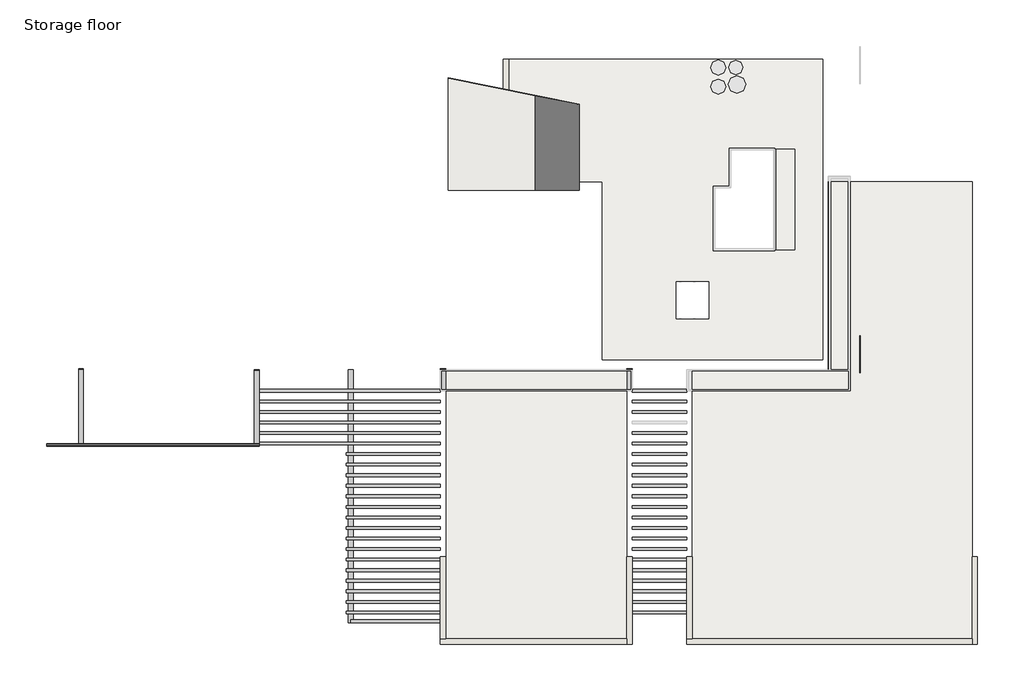
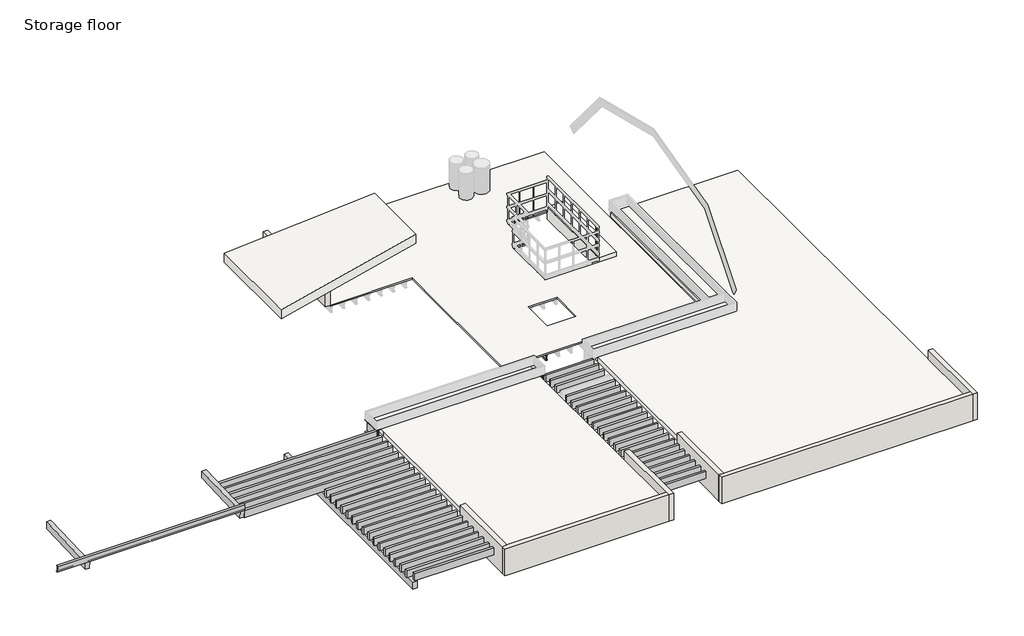
# One storey, part 1 of 2: 54 beams, 7 walls, 4 slabs, 1 roof.
"""IFC4 building model written with IfcOpenShell, lengths in millimetres."""

import ifcopenshell
import ifcopenshell.guid

model = None  # the IFC model being written
_history = None  # IfcOwnerHistory: only IFC2X3 demands one
_inside = {}  # id of a spatial element -> (the spatial element, [elements in it])
_under = {}  # id of a project, library or spatial element -> (it, [spatial elements below it])
_declared = {}  # id of a project -> (the project, [libraries it declares])
_typed = {}  # id of a type object -> (the type object, [elements of that type])
_made_of = {}  # id of a material, layer set ... -> (it, [elements and type objects made of it])


def new_model(schema):
    """Start an empty IFC model of exactly this schema.

    Asked for "IFC4X3", IfcOpenShell would pick the latest addendum, in which some entities
    have other attributes; the version numbers below select the first issue.
    IFC2X3 requires an IfcOwnerHistory on every rooted entity: one is made here for all.
    """
    global model, _history
    if schema == "IFC4X3":
        model = ifcopenshell.file(schema_version=(4, 3, 0, 0))
    else:
        model = ifcopenshell.file(schema=schema)
    _inside.clear()
    _under.clear()
    _declared.clear()
    _typed.clear()
    _made_of.clear()
    _history = None
    if model.schema == "IFC2X3":
        org = make("IfcOrganization", Name="unknown")
        user = make(
            "IfcPersonAndOrganization",
            ThePerson=make("IfcPerson", FamilyName="unknown"),
            TheOrganization=org,
        )
        app = make(
            "IfcApplication",
            ApplicationDeveloper=org,
            Version="unknown",
            ApplicationFullName="unknown",
            ApplicationIdentifier="unknown",
        )
        _history = make(
            "IfcOwnerHistory",
            OwningUser=user,
            OwningApplication=app,
            ChangeAction="ADDED",
            CreationDate=0,
        )
    return model


def make(cls, **values):
    """One entity of the class cls with the attributes given. An attribute that is None is left unset."""
    return model.create_entity(
        cls, **{name: value for name, value in values.items() if value is not None}
    )


def rooted(cls, **values):
    """An entity with a GlobalId (a new one), such as an element, a storey or a relation."""
    return make(cls, GlobalId=ifcopenshell.guid.new(), OwnerHistory=_history, **values)


def si_unit(unit_type, name, prefix=None):
    """IfcSIUnit, for example si_unit("LENGTHUNIT", "METRE", prefix="MILLI")."""
    return make("IfcSIUnit", UnitType=unit_type, Prefix=prefix, Name=name)


def assignment(units):
    """IfcUnitAssignment: the units of a project."""
    return None if units is None else make("IfcUnitAssignment", Units=units)


def point(xyz):
    """IfcCartesianPoint."""
    return None if xyz is None else make("IfcCartesianPoint", Coordinates=xyz)


def direction(xyz):
    """IfcDirection."""
    return None if xyz is None else make("IfcDirection", DirectionRatios=xyz)


def frame(location, z_axis=None, x_axis=None):
    """IfcAxis2Placement3D, a coordinate frame: its origin and axes. An axis left out is left unset."""
    return make(
        "IfcAxis2Placement3D",
        Location=point(location),
        Axis=direction(z_axis),
        RefDirection=direction(x_axis),
    )


def frame_2d(location, x_axis=None):
    """IfcAxis2Placement2D, a coordinate frame in the plane: its origin and x axis."""
    return make(
        "IfcAxis2Placement2D", Location=point(location), RefDirection=direction(x_axis)
    )


def origin():
    """The frame at (0, 0, 0) with its axes left unset."""
    return frame((0.0, 0.0, 0.0))


def place(relative_to, where):
    """IfcLocalPlacement: puts the frame where relative to a parent placement (None: the world)."""
    return make(
        "IfcLocalPlacement", PlacementRelTo=relative_to, RelativePlacement=where
    )


def context(
    kind, dimensions, precision=None, world=None, true_north=None, identifier=None
):
    """IfcGeometricRepresentationContext, for example the 3D "Model" context."""
    return make(
        "IfcGeometricRepresentationContext",
        ContextIdentifier=identifier,
        ContextType=kind,
        CoordinateSpaceDimension=dimensions,
        Precision=precision,
        WorldCoordinateSystem=world,
        TrueNorth=true_north,
    )


def project(units=None, contexts=None):
    """IfcProject with its units and contexts."""
    return rooted(
        "IfcProject",
        Name="project",
        RepresentationContexts=contexts,
        UnitsInContext=assignment(units),
    )


def spatial(cls, under=None, at=None, **own):
    """A site, building, storey or space (cls), placed at a placement, below another one or the project."""
    s = rooted(cls, ObjectPlacement=at, **own)
    if under is not None:
        _under.setdefault(under.id(), (under, []))[1].append(s)
    return s


def polyline(points):
    """IfcPolyline through the points."""
    return make("IfcPolyline", Points=[point(p) for p in points])


def circle_curve(where, radius):
    """IfcCircle in the frame where."""
    return make("IfcCircle", Position=where, Radius=radius)


def trimmed(basis, trim1, trim2, sense, master):
    """IfcTrimmedCurve: the piece of a basis curve between two trims."""
    return make(
        "IfcTrimmedCurve",
        BasisCurve=basis,
        Trim1=trim1,
        Trim2=trim2,
        SenseAgreement=sense,
        MasterRepresentation=master,
    )


def segment(curve, same_sense, transition):
    """IfcCompositeCurveSegment."""
    return make(
        "IfcCompositeCurveSegment",
        Transition=transition,
        SameSense=same_sense,
        ParentCurve=curve,
    )


def composite_curve(segments, self_intersect=None):
    """IfcCompositeCurve: segments joined end to end."""
    return make("IfcCompositeCurve", Segments=segments, SelfIntersect=self_intersect)


def outline(outer, holes=None, kind="AREA"):
    """IfcArbitraryClosedProfileDef: a profile drawn as a closed curve; with holes, ...WithVoids."""
    if holes is None:
        return make("IfcArbitraryClosedProfileDef", ProfileType=kind, OuterCurve=outer)
    return make(
        "IfcArbitraryProfileDefWithVoids",
        ProfileType=kind,
        OuterCurve=outer,
        InnerCurves=holes,
    )


def extrude(swept, where, along, depth):
    """IfcExtrudedAreaSolid: the profile swept, set in the frame where, extruded along a direction by depth."""
    return make(
        "IfcExtrudedAreaSolid",
        SweptArea=swept,
        Position=where,
        ExtrudedDirection=direction(along),
        Depth=depth,
    )


def faces_of(points, faces, orient=None, outer=None):
    """IfcFace entities. A face is a list of loops; a loop is a list of indices into points, from 0.

    orient and outer hold one flag for each loop. By default every Orientation is true, the
    first loop of a face is its IfcFaceOuterBound and the others are IfcFaceBound.
    """
    made = []
    for i, loops in enumerate(faces):
        bounds = []
        for j, loop in enumerate(loops):
            is_outer = j == 0 if outer is None else outer[i][j]
            bounds.append(
                make(
                    "IfcFaceOuterBound" if is_outer else "IfcFaceBound",
                    Bound=make("IfcPolyLoop", Polygon=[points[k] for k in loop]),
                    Orientation=True if orient is None else orient[i][j],
                )
            )
        made.append(make("IfcFace", Bounds=bounds))
    return made


def faceted_brep(points, faces, orient=None, outer=None, voids=None):
    """IfcFacetedBrep: a solid bounded by flat faces; with voids (closed shells), ...WithVoids."""
    shared = [point(p) for p in points]
    hull = make("IfcClosedShell", CfsFaces=faces_of(shared, faces, orient, outer))
    if voids is None:
        return make("IfcFacetedBrep", Outer=hull)
    return make(
        "IfcFacetedBrepWithVoids",
        Outer=hull,
        Voids=[
            make(cls, CfsFaces=faces_of(shared, fs, o, b)) for cls, fs, o, b in voids
        ],
    )


def shape(context_of_items, identifier, shape_type, items):
    """IfcShapeRepresentation: the items that make up one representation, for example the "Body"."""
    return make(
        "IfcShapeRepresentation",
        ContextOfItems=context_of_items,
        RepresentationIdentifier=identifier,
        RepresentationType=shape_type,
        Items=items,
    )


def source(mapping_origin, context_of_items, identifier, shape_type, items):
    """IfcRepresentationMap: a shape defined once, which mapped items show again and again."""
    return make(
        "IfcRepresentationMap",
        MappingOrigin=mapping_origin,
        MappedRepresentation=shape(context_of_items, identifier, shape_type, items),
    )


def transform(
    local_origin,
    x_axis=None,
    y_axis=None,
    z_axis=None,
    scale=None,
    scale2=None,
    scale3=None,
    uniform=True,
):
    """IfcCartesianTransformationOperator3D, or its non-uniform kind. x_axis, y_axis, z_axis: its Axis1, 2, 3."""
    if uniform:
        return make(
            "IfcCartesianTransformationOperator3D",
            Axis1=direction(x_axis),
            Axis2=direction(y_axis),
            LocalOrigin=point(local_origin),
            Scale=scale,
            Axis3=direction(z_axis),
        )
    return make(
        "IfcCartesianTransformationOperator3DnonUniform",
        Axis1=direction(x_axis),
        Axis2=direction(y_axis),
        LocalOrigin=point(local_origin),
        Scale=scale,
        Axis3=direction(z_axis),
        Scale2=scale2,
        Scale3=scale3,
    )


def mapped(mapping_source, mapping_target):
    """IfcMappedItem: shows the shape of a source again, moved by a transform."""
    return make(
        "IfcMappedItem", MappingSource=mapping_source, MappingTarget=mapping_target
    )


def made_of(thing, what):
    """Note that an element or type object is made of a material, layer set ...; save() writes the relation."""
    if what is not None:
        _made_of.setdefault(what.id(), (what, []))[1].append(thing)
    return thing


def element(
    cls,
    number,
    at=None,
    inside=None,
    cuts=None,
    type_object=None,
    material=None,
    context=None,
    identifier="Body",
    shape_type=None,
    held_by="IfcProductDefinitionShape",
    body=None,
    shapes=None,
    **own,
):
    """One element of the class cls, such as IfcWall. Its Tag is "e" and its number.

    at: its placement. inside: the storey or other place that contains it. cuts: it is an
    opening in that element (IfcRelVoidsElement). A single representation is given by context,
    identifier, shape_type and body (its items); several are given by shapes. held_by: the class
    of the entity that holds the representations. save() writes the other relations.
    """
    e = rooted(cls, Tag="e%d" % number, ObjectPlacement=at, **own)
    if body is not None:
        shapes = [shape(context, identifier, shape_type, body)]
    if shapes is not None:
        e.Representation = make(held_by, Representations=shapes)
    if inside is not None:
        _inside.setdefault(inside.id(), (inside, []))[1].append(e)
    if cuts is not None:
        rooted(
            "IfcRelVoidsElement", RelatingBuildingElement=cuts, RelatedOpeningElement=e
        )
    if type_object is not None:
        _typed.setdefault(type_object.id(), (type_object, []))[1].append(e)
    return made_of(e, material)


def aggregate(whole, parts):
    """IfcRelAggregates: a whole, such as a stair, and the parts it consists of."""
    return rooted("IfcRelAggregates", RelatingObject=whole, RelatedObjects=parts)


def save(model, path):
    """Write the relations noted so far, then the file.

    IfcRelAggregates (storeys below a building ...), IfcRelContainedInSpatialStructure (elements
    in a storey), IfcRelDefinesByType, IfcRelAssociatesMaterial and IfcRelDeclares: one each for
    every whole, place, type object, material and project.
    """
    for whole, parts in _under.values():
        aggregate(whole, parts)
    for where, things in _inside.values():
        rooted(
            "IfcRelContainedInSpatialStructure",
            RelatedElements=things,
            RelatingStructure=where,
        )
    for kind, things in _typed.values():
        rooted("IfcRelDefinesByType", RelatedObjects=things, RelatingType=kind)
    for what, things in _made_of.values():
        rooted("IfcRelAssociatesMaterial", RelatedObjects=things, RelatingMaterial=what)
    for by, libraries in _declared.values():
        rooted("IfcRelDeclares", RelatingContext=by, RelatedDefinitions=libraries)
    model.write(path)


def c_channel_c_3x8_0f191833(model_context):
    return source(origin(), model_context, "Body", "SweptSolid", [
        extrude(outline(composite_curve([segment(polyline([(-13.5128, 101.6), (44.9072, 101.6)]), True, "CONTINUOUS"), segment(trimmed(circle_curve(frame_2d((35.6108, 101.6)), 9.2964), [point((44.9072, 101.6))], [point((35.6108, 92.3036))], False, "CARTESIAN"), True, "CONTINUOUS"), segment(polyline([(35.6108, 92.3036), (-2.8702, 86.2088084), (-2.8702, -86.2088084), (35.6108, -92.3036)]), True, "CONTINUOUS"), segment(trimmed(circle_curve(frame_2d((35.6108, -101.6)), 9.2964), [point((35.6108, -92.3036))], [point((44.9072, -101.6))], False, "CARTESIAN"), True, "CONTINUOUS"), segment(polyline([(44.9072, -101.6), (-13.5128, -101.6), (-13.5128, 101.6)]), True, "CONTINUOUS")], self_intersect=False)), frame((-12252.325, 0.0, 0.0), z_axis=(1.0, 0.0, 0.0), x_axis=(0.0, 1.0, 0.0)), (0.0, 0.0, 1.0), 6108.7),
    ])


def plywood_web_joist_2_x_8_7c958bd9(model_context):
    return source(origin(), model_context, "Body", "SweptSolid", [
        extrude(outline(polyline([(-25.4, 101.6), (25.4, 101.6), (25.4, 63.5), (4.7625, 63.5), (4.7625, 69.85), (-4.7625, 69.85), (-4.7625, 63.5), (-25.4, 63.5), (-25.4, 101.6)])), frame((-4318.0, 0.0, 0.0), z_axis=(1.0, 0.0, 0.0), x_axis=(0.0, 1.0, 0.0)), (0.0, 0.0, 1.0), 8636.0),
        extrude(outline(polyline([(25.4, -63.5), (25.4, -101.6), (-25.4, -101.6), (-25.4, -63.5), (-4.7625, -63.5), (-4.7625, -69.1160374), (4.7625, -69.1160374), (4.7625, -63.5), (25.4, -63.5)])), frame((-4318.0, 0.0, 0.0), z_axis=(1.0, 0.0, 0.0), x_axis=(0.0, 1.0, 0.0)), (0.0, 0.0, 1.0), 8636.0),
        extrude(outline(polyline([(4318.0, 4.7625), (4318.0, -4.7625), (-4318.0, -4.7625), (-4318.0, 4.7625), (4318.0, 4.7625)])), frame((0.0, 0.0, -69.1160374), z_axis=(0.0, 0.0, 1.0), x_axis=(1.0, 0.0, 0.0)), (0.0, 0.0, 1.0), 138.9660374),
    ])


def timber_3x10_5e682144(model_context):
    return source(origin(), model_context, "Body", "SweptSolid", [
        extrude(outline(polyline([(1352.55, 38.1), (1352.55, -38.1), (-1352.55, -38.1), (-1352.55, 38.1), (1352.55, 38.1)])), frame((0.0, 0.0, -120.65), z_axis=(0.0, 0.0, 1.0), x_axis=(1.0, 0.0, 0.0)), (0.0, 0.0, 1.0), 241.3),
    ])


def timber_3x10_88a0bdfd(model_context):
    return source(origin(), model_context, "Body", "SweptSolid", [
        extrude(outline(polyline([(785.1325751, 38.1), (785.1325751, -38.1), (-785.1325751, -38.1), (-785.1325751, 38.1), (785.1325751, 38.1)])), frame((0.0, 0.0, -120.65), z_axis=(0.0, 0.0, 1.0), x_axis=(1.0, 0.0, 0.0)), (0.0, 0.0, 1.0), 241.3),
    ])


def timber_3x10_fcfe8c29(model_context):
    return source(origin(), model_context, "Body", "SweptSolid", [
        extrude(outline(polyline([(2603.5, 38.1), (2603.5, -38.1), (-2603.5, -38.1), (-2603.5, 38.1), (2603.5, 38.1)])), frame((0.0, 0.0, -120.65), z_axis=(0.0, 0.0, 1.0), x_axis=(1.0, 0.0, 0.0)), (0.0, 0.0, 1.0), 241.3),
    ])


def timber_3x10_eec112f8(model_context):
    return source(origin(), model_context, "Body", "SweptSolid", [
        extrude(outline(polyline([(2565.4, 38.1), (2565.4, -38.1), (-2641.6, -38.1), (-2641.6, 38.1), (2565.4, 38.1)])), frame((0.0, 0.0, -120.65), z_axis=(0.0, 0.0, 1.0), x_axis=(1.0, 0.0, 0.0)), (0.0, 0.0, 1.0), 241.3),
    ])


def timber_3x10_b3201cc8(model_context):
    return source(origin(), model_context, "Body", "SweptSolid", [
        extrude(outline(polyline([(1384.2999994, 38.1), (1384.2999994, -38.1), (-1197.0684633, -38.1), (-1197.0684633, 38.1), (1384.2999994, 38.1)])), frame((0.0, 0.0, -120.65), z_axis=(0.0, 0.0, 1.0), x_axis=(1.0, 0.0, 0.0)), (0.0, 0.0, 1.0), 241.3),
    ])


def timber_6x10_702de74f(model_context):
    return source(origin(), model_context, "Body", "SweptSolid", [
        extrude(outline(polyline([(1096.3279, 69.85), (1096.3279, -69.85), (-1065.1814977, -69.85), (-1065.1814977, 69.85), (1096.3279, 69.85)])), frame((0.0, 0.0, -120.65), z_axis=(0.0, 0.0, 1.0), x_axis=(1.0, 0.0, 0.0)), (0.0, 0.0, 1.0), 241.3),
    ])


def timber_6x10_97aa413e(model_context):
    return source(origin(), model_context, "Body", "SweptSolid", [
        extrude(outline(polyline([(1096.3279, 69.85), (1096.3279, -69.85), (-1091.5816749, -69.85), (-1091.5816749, 69.85), (1096.3279, 69.85)])), frame((0.0, 0.0, -120.65), z_axis=(0.0, 0.0, 1.0), x_axis=(1.0, 0.0, 0.0)), (0.0, 0.0, 1.0), 241.3),
    ])


def timber_6x10_01175893(model_context):
    return source(origin(), model_context, "Body", "SweptSolid", [
        extrude(outline(polyline([(1821.0853, 69.85), (1821.0853, -69.85), (-5454.65, -69.85), (-5454.65, 69.85), (1821.0853, 69.85)])), frame((0.0, 0.0, -120.65), z_axis=(0.0, 0.0, 1.0), x_axis=(1.0, 0.0, 0.0)), (0.0, 0.0, 1.0), 241.3),
    ])


def w_shapes_w_6x16_3_4_094122b6(model_context):
    return source(origin(), model_context, "Body", "SweptSolid", [
        extrude(outline(composite_curve([segment(polyline([(76.1964281, -203.073), (76.1964281, -212.725), (-76.2035719, -212.725), (-76.2035719, -203.073), (-10.5445719, -203.073)]), True, "CONTINUOUS"), segment(trimmed(circle_curve(frame_2d((-10.5445719, -195.453)), 7.62), [point((-10.5445719, -203.073))], [point((-2.9245719, -195.453))], True, "CARTESIAN"), True, "CONTINUOUS"), segment(polyline([(-2.9245719, -195.453), (-2.9245719, 195.453)]), True, "CONTINUOUS"), segment(trimmed(circle_curve(frame_2d((-10.5445719, 195.453)), 7.62), [point((-2.9245719, 195.453))], [point((-10.5445719, 203.073))], True, "CARTESIAN"), True, "CONTINUOUS"), segment(polyline([(-10.5445719, 203.073), (-76.2035719, 203.073), (-76.2035719, 212.725), (76.1964281, 212.725), (76.1964281, 203.073), (10.5374281, 203.073)]), True, "CONTINUOUS"), segment(trimmed(circle_curve(frame_2d((10.5374281, 195.453)), 7.62), [point((10.5374281, 203.073))], [point((2.9174281, 195.453))], True, "CARTESIAN"), True, "CONTINUOUS"), segment(polyline([(2.9174281, 195.453), (2.9174281, -195.453)]), True, "CONTINUOUS"), segment(trimmed(circle_curve(frame_2d((10.5374281, -195.453)), 7.62), [point((2.9174281, -195.453))], [point((10.5374281, -203.073))], True, "CARTESIAN"), True, "CONTINUOUS"), segment(polyline([(10.5374281, -203.073), (76.1964281, -203.073)]), True, "CONTINUOUS")], self_intersect=False)), frame((-315.8556375, 0.0, 0.0), z_axis=(1.0, 0.0, 0.0), x_axis=(0.0, 1.0, 0.0)), (0.0, 0.0, 1.0), 631.711275),
    ])


model = new_model("IFC4")

# Units and contexts
model_context = context("Model", 3, world=origin())
ifc_project = project(units=[si_unit("LENGTHUNIT", "METRE", prefix="MILLI")], contexts=[model_context])

# Site, building, storey
site = spatial("IfcSite", under=ifc_project)
building = spatial("IfcBuilding", under=site)
storey = spatial("IfcBuildingStorey", under=building, Name="Storage floor", Elevation=2832.1)

# Beams
placement = place(None, origin())
c_channel_c_3x8_shape = c_channel_c_3x8_0f191833(model_context)
element("IfcBeam", 1, ObjectType="C-Channel : C 3x8", at=placement, inside=storey, context=model_context, shape_type="MappedRepresentation", body=[
    mapped(c_channel_c_3x8_shape, transform((18838.0620052, 339.1116217, 2964.9027241), x_axis=(1.0, 0.0, 0.0), y_axis=(0.0, 0.9992458002577418, 0.03883079534680298), z_axis=(0.0, -0.03883079534680298, 0.9992458002577418))),
])
plywood_web_joist_2_x_8_shape = plywood_web_joist_2_x_8_7c958bd9(model_context)
element("IfcBeam", 2, ObjectType="Plywood Web Joist : 2 x 8", at=placement, inside=storey, context=model_context, shape_type="MappedRepresentation", body=[
    mapped(plywood_web_joist_2_x_8_shape, transform((23974.0792207, 7113.2615366, 2686.05), x_axis=(0.0, -1.0, 0.0), y_axis=(1.0, 0.0, 0.0), z_axis=(0.0, 0.0, 1.0))),
])
element("IfcBeam", 3, ObjectType="Plywood Web Joist : 2 x 8", at=placement, inside=storey, context=model_context, shape_type="MappedRepresentation", body=[
    mapped(plywood_web_joist_2_x_8_shape, transform((23567.6792207, 7113.2615366, 2686.05), x_axis=(0.0, -1.0, 0.0), y_axis=(1.0, 0.0, 0.0), z_axis=(0.0, 0.0, 1.0))),
])
element("IfcBeam", 4, ObjectType="Plywood Web Joist : 2 x 8", at=placement, inside=storey, context=model_context, shape_type="MappedRepresentation", body=[
    mapped(plywood_web_joist_2_x_8_shape, transform((23161.2792207, 7113.2615366, 2686.05), x_axis=(0.0, -1.0, 0.0), y_axis=(1.0, 0.0, 0.0), z_axis=(0.0, 0.0, 1.0))),
])
element("IfcBeam", 5, ObjectType="Plywood Web Joist : 2 x 8", at=placement, inside=storey, context=model_context, shape_type="MappedRepresentation", body=[
    mapped(plywood_web_joist_2_x_8_shape, transform((22754.8792207, 7113.2615366, 2686.05), x_axis=(0.0, -1.0, 0.0), y_axis=(1.0, 0.0, 0.0), z_axis=(0.0, 0.0, 1.0))),
])
timber_3x10_shape = timber_3x10_5e682144(model_context)
element("IfcBeam", 6, ObjectType="Timber : 3x10", at=placement, inside=storey, context=model_context, shape_type="MappedRepresentation", body=[
    mapped(timber_3x10_shape, transform((16548.8870052, 90.6164366, 2711.45), x_axis=(1.0, 0.0, 0.0), y_axis=(0.0, 1.0, 0.0), z_axis=(0.0, 0.0, 1.0))),
])
element("IfcBeam", 7, ObjectType="Timber : 3x10", at=placement, inside=storey, context=model_context, shape_type="MappedRepresentation", body=[
    mapped(timber_3x10_shape, transform((16548.8870052, -212.5392009, 2711.45), x_axis=(1.0, 0.0, 0.0), y_axis=(0.0, 1.0, 0.0), z_axis=(0.0, 0.0, 1.0))),
])
element("IfcBeam", 8, ObjectType="Timber : 3x10", at=placement, inside=storey, context=model_context, shape_type="MappedRepresentation", body=[
    mapped(timber_3x10_shape, transform((16548.8870052, -515.6948384, 2711.45), x_axis=(1.0, 0.0, 0.0), y_axis=(0.0, 1.0, 0.0), z_axis=(0.0, 0.0, 1.0))),
])
element("IfcBeam", 9, ObjectType="Timber : 3x10", at=placement, inside=storey, context=model_context, shape_type="MappedRepresentation", body=[
    mapped(timber_3x10_shape, transform((16548.8870052, -818.8504759, 2711.45), x_axis=(1.0, 0.0, 0.0), y_axis=(0.0, 1.0, 0.0), z_axis=(0.0, 0.0, 1.0))),
])
element("IfcBeam", 10, ObjectType="Timber : 3x10", at=placement, inside=storey, context=model_context, shape_type="MappedRepresentation", body=[
    mapped(timber_3x10_shape, transform((16548.8870052, -1122.0061134, 2711.45), x_axis=(1.0, 0.0, 0.0), y_axis=(0.0, 1.0, 0.0), z_axis=(0.0, 0.0, 1.0))),
])
element("IfcBeam", 11, ObjectType="Timber : 3x10", at=placement, inside=storey, context=model_context, shape_type="MappedRepresentation", body=[
    mapped(timber_3x10_shape, transform((16548.8870052, -1425.1617509, 2711.45), x_axis=(1.0, 0.0, 0.0), y_axis=(0.0, 1.0, 0.0), z_axis=(0.0, 0.0, 1.0))),
])
element("IfcBeam", 12, ObjectType="Timber : 3x10", at=placement, inside=storey, context=model_context, shape_type="MappedRepresentation", body=[
    mapped(timber_3x10_shape, transform((16548.8870052, -1728.3173884, 2711.45), x_axis=(1.0, 0.0, 0.0), y_axis=(0.0, 1.0, 0.0), z_axis=(0.0, 0.0, 1.0))),
])
element("IfcBeam", 13, ObjectType="Timber : 3x10", at=placement, inside=storey, context=model_context, shape_type="MappedRepresentation", body=[
    mapped(timber_3x10_shape, transform((16548.8870052, -2031.4730259, 2711.45), x_axis=(1.0, 0.0, 0.0), y_axis=(0.0, 1.0, 0.0), z_axis=(0.0, 0.0, 1.0))),
])
element("IfcBeam", 14, ObjectType="Timber : 3x10", at=placement, inside=storey, context=model_context, shape_type="MappedRepresentation", body=[
    mapped(timber_3x10_shape, transform((16548.8870052, -2334.6286634, 2711.45), x_axis=(1.0, 0.0, 0.0), y_axis=(0.0, 1.0, 0.0), z_axis=(0.0, 0.0, 1.0))),
])
element("IfcBeam", 15, ObjectType="Timber : 3x10", at=placement, inside=storey, context=model_context, shape_type="MappedRepresentation", body=[
    mapped(timber_3x10_shape, transform((16548.8870052, -2637.7843009, 2711.45), x_axis=(1.0, 0.0, 0.0), y_axis=(0.0, 1.0, 0.0), z_axis=(0.0, 0.0, 1.0))),
])
element("IfcBeam", 16, ObjectType="Timber : 3x10", at=placement, inside=storey, context=model_context, shape_type="MappedRepresentation", body=[
    mapped(timber_3x10_shape, transform((16548.8870052, -2940.9399384, 2711.45), x_axis=(1.0, 0.0, 0.0), y_axis=(0.0, 1.0, 0.0), z_axis=(0.0, 0.0, 1.0))),
])
element("IfcBeam", 17, ObjectType="Timber : 3x10", at=placement, inside=storey, context=model_context, shape_type="MappedRepresentation", body=[
    mapped(timber_3x10_shape, transform((16548.8870052, -3244.0955759, 2711.45), x_axis=(1.0, 0.0, 0.0), y_axis=(0.0, 1.0, 0.0), z_axis=(0.0, 0.0, 1.0))),
])
element("IfcBeam", 18, ObjectType="Timber : 3x10", at=placement, inside=storey, context=model_context, shape_type="MappedRepresentation", body=[
    mapped(timber_3x10_shape, transform((16548.8870052, -3547.2512134, 2711.45), x_axis=(1.0, 0.0, 0.0), y_axis=(0.0, 1.0, 0.0), z_axis=(0.0, 0.0, 1.0))),
])
element("IfcBeam", 19, ObjectType="Timber : 3x10", at=placement, inside=storey, context=model_context, shape_type="MappedRepresentation", body=[
    mapped(timber_3x10_shape, transform((16548.8870052, -3850.4068509, 2711.45), x_axis=(1.0, 0.0, 0.0), y_axis=(0.0, 1.0, 0.0), z_axis=(0.0, 0.0, 1.0))),
])
element("IfcBeam", 20, ObjectType="Timber : 3x10", at=placement, inside=storey, context=model_context, shape_type="MappedRepresentation", body=[
    mapped(timber_3x10_shape, transform((16548.8870052, -4153.5624884, 2711.45), x_axis=(1.0, 0.0, 0.0), y_axis=(0.0, 1.0, 0.0), z_axis=(0.0, 0.0, 1.0))),
])
element("IfcBeam", 21, ObjectType="Timber : 3x10", at=placement, inside=storey, context=model_context, shape_type="MappedRepresentation", body=[
    mapped(timber_3x10_shape, transform((16548.8870052, -4456.7181259, 2711.45), x_axis=(1.0, 0.0, 0.0), y_axis=(0.0, 1.0, 0.0), z_axis=(0.0, 0.0, 1.0))),
])
timber_3x10_2_shape = timber_3x10_88a0bdfd(model_context)
element("IfcBeam", 22, ObjectType="Timber : 3x10", at=placement, inside=storey, context=model_context, shape_type="MappedRepresentation", body=[
    mapped(timber_3x10_2_shape, transform((24192.0195803, 1606.3946241, 2711.45), x_axis=(1.0, 0.0, 0.0), y_axis=(0.0, 1.0, 0.0), z_axis=(0.0, 0.0, 1.0))),
])
element("IfcBeam", 23, ObjectType="Timber : 3x10", at=placement, inside=storey, context=model_context, shape_type="MappedRepresentation", body=[
    mapped(timber_3x10_2_shape, transform((24192.0195803, 1303.2389866, 2711.45), x_axis=(1.0, 0.0, 0.0), y_axis=(0.0, 1.0, 0.0), z_axis=(0.0, 0.0, 1.0))),
])
element("IfcBeam", 24, ObjectType="Timber : 3x10", at=placement, inside=storey, context=model_context, shape_type="MappedRepresentation", body=[
    mapped(timber_3x10_2_shape, transform((24192.0195803, 696.9277116, 2711.45), x_axis=(1.0, 0.0, 0.0), y_axis=(0.0, 1.0, 0.0), z_axis=(0.0, 0.0, 1.0))),
])
element("IfcBeam", 25, ObjectType="Timber : 3x10", at=placement, inside=storey, context=model_context, shape_type="MappedRepresentation", body=[
    mapped(timber_3x10_2_shape, transform((24192.0195803, 393.7720741, 2711.45), x_axis=(1.0, 0.0, 0.0), y_axis=(0.0, 1.0, 0.0), z_axis=(0.0, 0.0, 1.0))),
])
element("IfcBeam", 26, ObjectType="Timber : 3x10", at=placement, inside=storey, context=model_context, shape_type="MappedRepresentation", body=[
    mapped(timber_3x10_2_shape, transform((24192.0195803, 90.6164366, 2711.45), x_axis=(1.0, 0.0, 0.0), y_axis=(0.0, 1.0, 0.0), z_axis=(0.0, 0.0, 1.0))),
])
element("IfcBeam", 27, ObjectType="Timber : 3x10", at=placement, inside=storey, context=model_context, shape_type="MappedRepresentation", body=[
    mapped(timber_3x10_2_shape, transform((24192.0195803, -212.5392009, 2711.45), x_axis=(1.0, 0.0, 0.0), y_axis=(0.0, 1.0, 0.0), z_axis=(0.0, 0.0, 1.0))),
])
element("IfcBeam", 28, ObjectType="Timber : 3x10", at=placement, inside=storey, context=model_context, shape_type="MappedRepresentation", body=[
    mapped(timber_3x10_2_shape, transform((24192.0195803, -515.6948384, 2711.45), x_axis=(1.0, 0.0, 0.0), y_axis=(0.0, 1.0, 0.0), z_axis=(0.0, 0.0, 1.0))),
])
element("IfcBeam", 29, ObjectType="Timber : 3x10", at=placement, inside=storey, context=model_context, shape_type="MappedRepresentation", body=[
    mapped(timber_3x10_2_shape, transform((24192.0195803, -818.8504759, 2711.45), x_axis=(1.0, 0.0, 0.0), y_axis=(0.0, 1.0, 0.0), z_axis=(0.0, 0.0, 1.0))),
])
element("IfcBeam", 30, ObjectType="Timber : 3x10", at=placement, inside=storey, context=model_context, shape_type="MappedRepresentation", body=[
    mapped(timber_3x10_2_shape, transform((24192.0195803, -1122.0061134, 2711.45), x_axis=(1.0, 0.0, 0.0), y_axis=(0.0, 1.0, 0.0), z_axis=(0.0, 0.0, 1.0))),
])
element("IfcBeam", 31, ObjectType="Timber : 3x10", at=placement, inside=storey, context=model_context, shape_type="MappedRepresentation", body=[
    mapped(timber_3x10_2_shape, transform((24192.0195803, -1425.1617509, 2711.45), x_axis=(1.0, 0.0, 0.0), y_axis=(0.0, 1.0, 0.0), z_axis=(0.0, 0.0, 1.0))),
])
element("IfcBeam", 32, ObjectType="Timber : 3x10", at=placement, inside=storey, context=model_context, shape_type="MappedRepresentation", body=[
    mapped(timber_3x10_2_shape, transform((24192.0195803, -1728.3173884, 2711.45), x_axis=(1.0, 0.0, 0.0), y_axis=(0.0, 1.0, 0.0), z_axis=(0.0, 0.0, 1.0))),
])
element("IfcBeam", 33, ObjectType="Timber : 3x10", at=placement, inside=storey, context=model_context, shape_type="MappedRepresentation", body=[
    mapped(timber_3x10_2_shape, transform((24192.0195803, -2031.4730259, 2711.45), x_axis=(1.0, 0.0, 0.0), y_axis=(0.0, 1.0, 0.0), z_axis=(0.0, 0.0, 1.0))),
])
element("IfcBeam", 34, ObjectType="Timber : 3x10", at=placement, inside=storey, context=model_context, shape_type="MappedRepresentation", body=[
    mapped(timber_3x10_2_shape, transform((24192.0195803, -2334.6286634, 2711.45), x_axis=(1.0, 0.0, 0.0), y_axis=(0.0, 1.0, 0.0), z_axis=(0.0, 0.0, 1.0))),
])
element("IfcBeam", 35, ObjectType="Timber : 3x10", at=placement, inside=storey, context=model_context, shape_type="MappedRepresentation", body=[
    mapped(timber_3x10_2_shape, transform((24192.0195803, -2637.7843009, 2711.45), x_axis=(1.0, 0.0, 0.0), y_axis=(0.0, 1.0, 0.0), z_axis=(0.0, 0.0, 1.0))),
])
element("IfcBeam", 36, ObjectType="Timber : 3x10", at=placement, inside=storey, context=model_context, shape_type="MappedRepresentation", body=[
    mapped(timber_3x10_2_shape, transform((24192.0195803, -2940.9399384, 2711.45), x_axis=(1.0, 0.0, 0.0), y_axis=(0.0, 1.0, 0.0), z_axis=(0.0, 0.0, 1.0))),
])
element("IfcBeam", 37, ObjectType="Timber : 3x10", at=placement, inside=storey, context=model_context, shape_type="MappedRepresentation", body=[
    mapped(timber_3x10_2_shape, transform((24192.0195803, -3244.0955759, 2711.45), x_axis=(1.0, 0.0, 0.0), y_axis=(0.0, 1.0, 0.0), z_axis=(0.0, 0.0, 1.0))),
])
element("IfcBeam", 38, ObjectType="Timber : 3x10", at=placement, inside=storey, context=model_context, shape_type="MappedRepresentation", body=[
    mapped(timber_3x10_2_shape, transform((24192.0195803, -3547.2512134, 2711.45), x_axis=(1.0, 0.0, 0.0), y_axis=(0.0, 1.0, 0.0), z_axis=(0.0, 0.0, 1.0))),
])
element("IfcBeam", 39, ObjectType="Timber : 3x10", at=placement, inside=storey, context=model_context, shape_type="MappedRepresentation", body=[
    mapped(timber_3x10_2_shape, transform((24192.0195803, -3850.4068509, 2711.45), x_axis=(1.0, 0.0, 0.0), y_axis=(0.0, 1.0, 0.0), z_axis=(0.0, 0.0, 1.0))),
])
element("IfcBeam", 40, ObjectType="Timber : 3x10", at=placement, inside=storey, context=model_context, shape_type="MappedRepresentation", body=[
    mapped(timber_3x10_2_shape, transform((24192.0195803, -4153.5624884, 2711.45), x_axis=(1.0, 0.0, 0.0), y_axis=(0.0, 1.0, 0.0), z_axis=(0.0, 0.0, 1.0))),
])
element("IfcBeam", 41, ObjectType="Timber : 3x10", at=placement, inside=storey, context=model_context, shape_type="MappedRepresentation", body=[
    mapped(timber_3x10_2_shape, transform((24192.0195803, -4456.7181259, 2711.45), x_axis=(1.0, 0.0, 0.0), y_axis=(0.0, 1.0, 0.0), z_axis=(0.0, 0.0, 1.0))),
])
element("IfcBeam", 42, ObjectType="Timber : 3x10", at=placement, inside=storey, context=model_context, shape_type="MappedRepresentation", body=[
    mapped(timber_3x10_2_shape, transform((24192.0195803, 1909.5502616, 2711.45), x_axis=(1.0, 0.0, 0.0), y_axis=(0.0, 1.0, 0.0), z_axis=(0.0, 0.0, 1.0))),
])
timber_3x10_3_shape = timber_3x10_fcfe8c29(model_context)
element("IfcBeam", 43, ObjectType="Timber : 3x10", at=placement, inside=storey, context=model_context, shape_type="MappedRepresentation", body=[
    mapped(timber_3x10_3_shape, transform((15297.9370052, 1606.3946241, 2711.45), x_axis=(1.0, 0.0, 0.0), y_axis=(0.0, 1.0, 0.0), z_axis=(0.0, 0.0, 1.0))),
])
element("IfcBeam", 44, ObjectType="Timber : 3x10", at=placement, inside=storey, context=model_context, shape_type="MappedRepresentation", body=[
    mapped(timber_3x10_3_shape, transform((15297.9370052, 1303.2389866, 2711.45), x_axis=(1.0, 0.0, 0.0), y_axis=(0.0, 1.0, 0.0), z_axis=(0.0, 0.0, 1.0))),
])
element("IfcBeam", 45, ObjectType="Timber : 3x10", at=placement, inside=storey, context=model_context, shape_type="MappedRepresentation", body=[
    mapped(timber_3x10_3_shape, transform((15297.9370052, 1000.0833491, 2711.45), x_axis=(1.0, 0.0, 0.0), y_axis=(0.0, 1.0, 0.0), z_axis=(0.0, 0.0, 1.0))),
])
element("IfcBeam", 46, ObjectType="Timber : 3x10", at=placement, inside=storey, context=model_context, shape_type="MappedRepresentation", body=[
    mapped(timber_3x10_3_shape, transform((15297.9370052, 696.9277116, 2711.45), x_axis=(1.0, 0.0, 0.0), y_axis=(0.0, 1.0, 0.0), z_axis=(0.0, 0.0, 1.0))),
])
element("IfcBeam", 47, ObjectType="Timber : 3x10", at=placement, inside=storey, context=model_context, shape_type="MappedRepresentation", body=[
    mapped(timber_3x10_3_shape, transform((15297.9370052, 393.7720741, 2711.45), x_axis=(1.0, 0.0, 0.0), y_axis=(0.0, 1.0, 0.0), z_axis=(0.0, 0.0, 1.0))),
])
timber_3x10_4_shape = timber_3x10_eec112f8(model_context)
element("IfcBeam", 48, ObjectType="Timber : 3x10", at=placement, inside=storey, context=model_context, shape_type="MappedRepresentation", body=[
    mapped(timber_3x10_4_shape, transform((15336.0370052, 1909.5502616, 2711.45), x_axis=(1.0, 0.0, 0.0), y_axis=(0.0, 1.0, 0.0), z_axis=(0.0, 0.0, 1.0))),
])
timber_3x10_5_shape = timber_3x10_b3201cc8(model_context)
element("IfcBeam", 49, ObjectType="Timber : 3x10", at=placement, inside=storey, context=model_context, shape_type="MappedRepresentation", body=[
    mapped(timber_3x10_5_shape, transform((16704.3685419, -4709.0737634, 2711.45), x_axis=(-1.0, 0.0, 0.0), y_axis=(0.0, -1.0, 0.0), z_axis=(0.0, 0.0, 1.0))),
])
timber_6x10_shape = timber_6x10_702de74f(model_context)
element("IfcBeam", 50, ObjectType="Timber : 6x10", at=placement, inside=storey, context=model_context, shape_type="MappedRepresentation", body=[
    mapped(timber_6x10_shape, transform((12624.5870052, 1444.2456915, 2787.7151492), x_axis=(0.0, -0.9992458002577417, -0.03883079534680293), y_axis=(1.0, 0.0, 0.0), z_axis=(0.0, -0.038830795346802935, 0.9992458002577418))),
])
timber_6x10_2_shape = timber_6x10_97aa413e(model_context)
element("IfcBeam", 51, ObjectType="Timber : 6x10", at=placement, inside=storey, context=model_context, shape_type="MappedRepresentation", body=[
    mapped(timber_6x10_2_shape, transform((7576.3370052, 1444.2456915, 2787.7151492), x_axis=(0.0, -0.9992458002577417, -0.03883079534680302), y_axis=(1.0, 0.0, 0.0), z_axis=(0.0, -0.038830795346803025, 0.9992458002577418))),
])
timber_6x10_3_shape = timber_6x10_01175893(model_context)
element("IfcBeam", 52, ObjectType="Timber : 6x10", at=placement, inside=storey, context=model_context, shape_type="MappedRepresentation", body=[
    mapped(timber_6x10_3_shape, transform((15320.0685419, -2938.7884634, 2457.45), x_axis=(0.0, -1.0, 0.0), y_axis=(1.0, 0.0, 0.0), z_axis=(0.0, 0.0, 1.0))),
])
w_shapes_w_6x16_3_4_shape = w_shapes_w_6x16_3_4_094122b6(model_context)
element("IfcBeam", 53, ObjectType="W Shapes : W 6X16 3/4", at=placement, inside=storey, context=model_context, shape_type="MappedRepresentation", body=[
    mapped(w_shapes_w_6x16_3_4_shape, transform((17977.6370052, 2225.4058991, 2619.371825), x_axis=(0.0, -1.0, 0.0), y_axis=(1.0, 0.0, 0.0), z_axis=(0.0, 0.0, 1.0))),
])
element("IfcBeam", 54, ObjectType="W Shapes : W 6X16 3/4", at=placement, inside=storey, context=model_context, shape_type="MappedRepresentation", body=[
    mapped(w_shapes_w_6x16_3_4_shape, transform((23330.6870052, 2225.4058991, 2619.371825), x_axis=(0.0, -1.0, 0.0), y_axis=(1.0, 0.0, 0.0), z_axis=(0.0, 0.0, 1.0))),
])

# Roof
element("IfcRoof", 55, ObjectType="Generic - 12\"", at=placement, inside=storey, context=model_context, shape_type="Brep", body=[
    faceted_brep([(22524.2370052, 7672.0615366, 4186.3004245), (18130.0334333, 7672.0615366, 3116.0032609), (18130.0334333, 10896.6893622, 3116.0032609), (22524.2370052, 10004.7750592, 4186.3004245), (18130.0334333, 7672.0615366, 3429.714351), (22524.2370052, 7672.0615366, 4500.0115147), (22524.2370052, 9990.1341782, 4500.0115147), (18130.0334333, 10882.0484812, 3429.714351)], [[[0, 1, 2, 3]], [[4, 5, 6, 7]], [[1, 4, 7, 2]], [[1, 0, 5, 4]], [[5, 0, 3, 6]], [[3, 2, 7, 6]]]),
])

# Slabs
element("IfcSlab", 56, ObjectType="Generic - 6\"", at=placement, inside=storey, context=model_context, shape_type="SweptSolid", body=[
    extrude(outline(polyline([(23254.4870052, -5217.0737634), (18066.5370052, -5217.0737634), (18066.5370052, 1753.8615366), (18066.5370052, 2515.8615366), (23254.4870052, 2515.8615366), (23254.4870052, 1753.8615366), (23254.4870052, -5217.0737634)])), frame((0.0, 0.0, 2679.7), z_axis=(0.0, 0.0, 1.0), x_axis=(1.0, 0.0, 0.0)), (0.0, 0.0, 1.0), 152.4),
])
element("IfcSlab", 57, ObjectType="Generic - 6\"", at=placement, inside=storey, context=model_context, shape_type="SweptSolid", body=[
    extrude(outline(polyline([(33173.1870052, -5217.0737634), (25129.5521553, -5217.0737634), (25129.5521553, 1906.2615366), (25129.5521553, 2515.8615366), (29032.9870052, 2515.8615366), (29032.9870052, 7913.3615366), (29820.3870052, 7913.3615366), (33173.1870052, 7913.3615366), (33173.1870052, -5217.0737634)])), frame((0.0, 0.0, 2679.7), z_axis=(0.0, 0.0, 1.0), x_axis=(1.0, 0.0, 0.0)), (0.0, 0.0, 1.0), 152.4),
])
element("IfcSlab", 58, ObjectType="Wood Joist 10\" - Wood Finish 2", at=placement, inside=storey, context=model_context, shape_type="SweptSolid", body=[
    extrude(outline(polyline([(19863.5870052, 11431.2615366), (28880.5870052, 11431.2615366), (28880.5870052, 2795.2615366), (22549.6370052, 2795.2615366), (22549.6370052, 7913.3615366), (19863.5870052, 7913.3615366), (19863.5870052, 11431.2615366)]), holes=[polyline([(28074.1370052, 8853.1615366), (26219.9370052, 8853.1615366), (26219.9370052, 7760.9615366), (25756.3870052, 7760.9615366), (25756.3870052, 5963.9115366), (28074.1370052, 5963.9115366), (28074.1370052, 8853.1615366)]), polyline([(25611.8964683, 5040.1381415), (24672.0964683, 5040.1381415), (24672.0964683, 3973.3381415), (25611.8964683, 3973.3381415), (25611.8964683, 5040.1381415)])]), frame((0.0, 0.0, 2787.65), z_axis=(0.0, 0.0, 1.0), x_axis=(1.0, 0.0, 0.0)), (0.0, 0.0, 1.0), 44.45),
])
element("IfcSlab", 59, ObjectType="Wood Joist 16\" - Wood Finish", at=placement, inside=storey, context=model_context, shape_type="SweptSolid", body=[
    extrude(outline(polyline([(27502.6370052, 8853.1615366), (28074.1370052, 8853.1615366), (28074.1370052, 5963.9115366), (27502.6370052, 5963.9115366), (27502.6370052, 8853.1615366)])), frame((0.0, 0.0, 2559.05), z_axis=(0.0, 0.0, 1.0), x_axis=(1.0, 0.0, 0.0)), (0.0, 0.0, 1.0), 425.45),
])

# Walls
element("IfcWall", 60, ObjectType="Generic - 6\"", at=placement, inside=storey, context=model_context, shape_type="Brep", body=[
    faceted_brep([(19711.1870052, 11431.2615366, 2832.1), (19711.1870052, 7913.3615366, 2832.1), (19711.1870052, 7913.3615366, 3501.1251961), (19711.1870052, 10575.7544162, 3501.1251961), (19711.1870052, 10575.7544162, 3285.2356146), (19711.1870052, 11431.2615366, 3285.2356146), (19863.5870052, 11431.2615366, 2832.1), (19863.5870052, 11431.2615366, 3285.2356146), (19863.5870052, 10544.8209973, 3285.2356146), (19863.5870052, 10544.8209973, 3538.2452988), (19863.5870052, 7913.3615366, 3538.2452988), (19863.5870052, 7913.3615366, 2832.1)], [[[0, 1, 2, 3, 4, 5]], [[6, 7, 8, 9, 10, 11]], [[1, 0, 6, 11]], [[2, 1, 11, 10]], [[0, 5, 7, 6]], [[5, 4, 8, 7]], [[3, 9, 8, 4]], [[3, 2, 10, 9]]]),
])
element("IfcWall", 61, ObjectType="Generic - 6\" wood", at=placement, inside=storey, context=model_context, shape_type="Brep", body=[
    faceted_brep([(33173.1870052, -2931.0737634, 2239.16875), (33173.1870052, -4683.6737634, 2239.16875), (33173.1870052, -5217.0737634, 2239.16875), (33173.1870052, -5369.4737634, 2239.16875), (33173.1870052, -5369.4737634, 3153.56875), (33173.1870052, -5217.0737634, 3153.56875), (33173.1870052, -2854.8737634, 3153.56875), (33173.1870052, -2854.8737634, 3153.3582813), (33173.1870052, -2854.8737634, 2679.7), (33173.1870052, -2931.0737634, 2679.7), (33325.5870052, -2931.0737634, 2239.16875), (33325.5870052, -2931.0737634, 2679.7), (33325.5870052, -2854.8737634, 2679.7), (33325.5870052, -2854.8737634, 3153.3582813), (33325.5870052, -2854.8737634, 3153.56875), (33325.5870052, -5369.4737634, 3153.56875), (33325.5870052, -5369.4737634, 2239.16875), (33325.5870052, -4683.6737634, 2239.16875)], [[[0, 1, 2, 3, 4, 5, 6, 7, 8, 9]], [[10, 11, 12, 13, 14, 15, 16, 17]], [[3, 2, 1, 0, 10, 17, 16]], [[6, 5, 4, 15, 14]], [[4, 3, 16, 15]], [[8, 7, 6, 14, 13, 12]], [[8, 12, 11, 9]], [[0, 9, 11, 10]]]),
])
element("IfcWall", 62, ObjectType="Generic - 6\" wood", at=placement, inside=storey, context=model_context, shape_type="Brep", body=[
    faceted_brep([(33173.1870052, -5217.0737634, 2239.16875), (25129.5521553, -5217.0737634, 2239.16875), (24977.1521553, -5217.0737634, 2239.16875), (24977.1521553, -5217.0737634, 3153.56875), (25129.5521553, -5217.0737634, 3153.56875), (33173.1870052, -5217.0737634, 3153.56875), (33173.1870052, -5369.4737634, 2239.16875), (33173.1870052, -5369.4737634, 3153.56875), (24977.1521553, -5369.4737634, 3153.56875), (24977.1521553, -5369.4737634, 2239.16875), (25129.5521553, -5369.4737634, 2239.16875)], [[[0, 1, 2, 3, 4, 5]], [[6, 7, 8, 9, 10]], [[2, 1, 0, 6, 10, 9]], [[5, 4, 3, 8, 7]], [[0, 5, 7, 6]], [[3, 2, 9, 8]]]),
])
element("IfcWall", 63, ObjectType="Generic - 6\" wood", at=placement, inside=storey, context=model_context, shape_type="Brep", body=[
    faceted_brep([(24977.1521553, -2931.0737634, 2239.16875), (24977.1521553, -4683.6737634, 2239.16875), (24977.1521553, -5217.0737634, 2239.16875), (24977.1521553, -5217.0737634, 3153.56875), (24977.1521553, -2854.8737634, 3153.56875), (24977.1521553, -2854.8737634, 3153.3582813), (24977.1521553, -2854.8737634, 2679.7), (24977.1521553, -2931.0737634, 2679.7), (25129.5521553, -2931.0737634, 2239.16875), (25129.5521553, -2931.0737634, 2679.7), (25129.5521553, -2854.8737634, 2679.7), (25129.5521553, -2854.8737634, 3153.3582813), (25129.5521553, -2854.8737634, 3153.56875), (25129.5521553, -5217.0737634, 3153.56875), (25129.5521553, -5217.0737634, 2239.16875), (25129.5521553, -4683.6737634, 2239.16875)], [[[0, 1, 2, 3, 4, 5, 6, 7]], [[8, 9, 10, 11, 12, 13, 14, 15]], [[2, 1, 0, 8, 15, 14]], [[4, 3, 13, 12]], [[3, 2, 14, 13]], [[6, 5, 4, 12, 11, 10]], [[6, 10, 9, 7]], [[0, 7, 9, 8]]]),
])
element("IfcWall", 64, ObjectType="Generic - 6\" wood", at=placement, inside=storey, context=model_context, shape_type="Brep", body=[
    faceted_brep([(23254.4870052, -2931.0737634, 2239.16875), (23254.4870052, -4683.6737634, 2239.16875), (23254.4870052, -5217.0737634, 2239.16875), (23254.4870052, -5369.4737634, 2239.16875), (23254.4870052, -5369.4737634, 3153.56875), (23254.4870052, -5217.0737634, 3153.56875), (23254.4870052, -2854.8737634, 3153.56875), (23254.4870052, -2854.8737634, 3153.3582813), (23254.4870052, -2854.8737634, 2679.7), (23254.4870052, -2931.0737634, 2679.7), (23406.8870052, -2931.0737634, 2239.16875), (23406.8870052, -2931.0737634, 2679.7), (23406.8870052, -2854.8737634, 2679.7), (23406.8870052, -2854.8737634, 3153.3582813), (23406.8870052, -2854.8737634, 3153.56875), (23406.8870052, -5369.4737634, 3153.56875), (23406.8870052, -5369.4737634, 2239.16875), (23406.8870052, -4683.6737634, 2239.16875)], [[[0, 1, 2, 3, 4, 5, 6, 7, 8, 9]], [[10, 11, 12, 13, 14, 15, 16, 17]], [[3, 2, 1, 0, 10, 17, 16]], [[6, 5, 4, 15, 14]], [[8, 7, 6, 14, 13, 12]], [[8, 12, 11, 9]], [[0, 9, 11, 10]], [[4, 3, 16, 15]]]),
])
element("IfcWall", 65, ObjectType="Generic - 6\" wood", at=placement, inside=storey, context=model_context, shape_type="Brep", body=[
    faceted_brep([(23254.4870052, -5217.0737634, 2239.16875), (18053.8370052, -5217.0737634, 2239.16875), (17901.4370052, -5217.0737634, 2239.16875), (17901.4370052, -5217.0737634, 3153.56875), (18053.8370052, -5217.0737634, 3153.56875), (23254.4870052, -5217.0737634, 3153.56875), (23254.4870052, -5369.4737634, 2239.16875), (23254.4870052, -5369.4737634, 3153.56875), (17901.4370052, -5369.4737634, 3153.56875), (17901.4370052, -5369.4737634, 2239.16875), (18053.8370052, -5369.4737634, 2239.16875)], [[[0, 1, 2, 3, 4, 5]], [[6, 7, 8, 9, 10]], [[2, 1, 0, 6, 10, 9]], [[5, 4, 3, 8, 7]], [[0, 5, 7, 6]], [[3, 2, 9, 8]]]),
])
element("IfcWall", 66, ObjectType="Generic - 6\" wood", at=placement, inside=storey, context=model_context, shape_type="Brep", body=[
    faceted_brep([(18053.8370052, -5217.0737634, 2239.16875), (18053.8370052, -4683.6737634, 2239.16875), (18053.8370052, -2931.0737634, 2239.16875), (18053.8370052, -2931.0737634, 2679.7), (18053.8370052, -2854.8737634, 2679.7), (18053.8370052, -2854.8737634, 3153.3582813), (18053.8370052, -2854.8737634, 3153.56875), (18053.8370052, -5217.0737634, 3153.56875), (17901.4370052, -5217.0737634, 2239.16875), (17901.4370052, -5217.0737634, 3153.56875), (17901.4370052, -2854.8737634, 3153.56875), (17901.4370052, -2854.8737634, 3153.3582813), (17901.4370052, -2854.8737634, 2679.7), (17901.4370052, -2931.0737634, 2679.7), (17901.4370052, -2931.0737634, 2239.16875), (17901.4370052, -4683.6737634, 2239.16875)], [[[0, 1, 2, 3, 4, 5, 6, 7]], [[8, 9, 10, 11, 12, 13, 14, 15]], [[2, 1, 0, 8, 15, 14]], [[7, 6, 10, 9]], [[0, 7, 9, 8]], [[6, 5, 4, 12, 11, 10]], [[12, 4, 3, 13]], [[3, 2, 14, 13]]]),
])

save(model, "model.ifc")

# Revit data of these elements
# Project information
#   Project Issue Date = "Issue Date"
#   Project Status = "Project Status"
#   Client Name = "Owner"
#   Project Address = "Enter address here"
#   Project Name = "Project Name"
#   Project Number = "Project Number"
# Type "C-Channel : C 3x8"
#   Assembly Code = "B10"
#   W = 14.7
#   Length [instance default] = 5' - 0"
#   bf = 0' - 2.3"
#   d = 0' - 8"
#   tf = 0' - 0.366"
#   tw = 0' - 0.419"
#   x = 0' - 0.532"
#   A = 0.0300694 SF
#   Structural Material [instance default] = Steel ASTM A36
# Type "Plywood Web Joist : 2 x 8"
#   Assembly Code = "B10"
#   Length [instance default] = 5' - 0"
#   b = 0' - 2"
#   d = 0' - 8"
#   Structural Material [instance default] = Softwood, Lumber
# Type "Timber : 3x10"
#   Assembly Code = "B10"
#   A = 0.362847 SF
#   Length [instance default] = 5' - 0"
#   b = 0' - 3"
#   d = 0' - 9 1/2"
#   Structural Material [instance default] = Softwood, Lumber
# Type "Timber : 6x10"
#   Assembly Code = "B10"
#   A = 0.362847 SF
#   Length [instance default] = 5' - 0"
#   b = 0' - 5 1/2"
#   d = 0' - 9 1/2"
#   Structural Material [instance default] = Softwood, Lumber
# Type "W Shapes : W 6X16 3/4"
#   Section Name Key = "W12x26"
#   Assembly Code = "B10"
#   Width = 152.4 mm
#   Web Thickness = 5.842 mm
#   Web Fillet = 7.62 mm
#   Warping Constant = 163001.3 cm⁶
#   Torsional Moment of Inertia = 12.4869 cm⁴
#   Section Area = 7.65 in²
#   Plastic Modulus weak axis = 0.00472801 (stored number, unit not read)
#   Plastic Modulus strong axis = 0.0215278 (stored number, unit not read)
#   Perimeter = 15.0571 m²/m
#   Nominal Weight = 379.441 N/m
#   Moment of Inertia weak axis = 720.08 cm⁴
#   Moment of Inertia strong axis = 8491.12 cm⁴
#   Height = 425.45 mm
#   Flange Thickness = 9.652 mm
#   Elastic Modulus weak axis = 0.00309028 (stored number, unit not read)
#   Elastic Modulus strong axis = 0.0193287 (stored number, unit not read)
#   Centroid Vertical = 212.725 mm
#   Centroid Horizontal = 76.2 mm
#   Length [instance default] = 5' - 0"
#   Structural Material [instance default] = Steel ASTM A992
#   Principal Axes Angle = 0
# Type "Generic - 12\""
#   Assembly Code = "B1020"
#   Layers, outside or top first: 1' - 0" no material (function 1)
# Type "Generic - 6\""
#   Assembly Code = "B1010"
#   Function = 0
#   Layers, outside or top first: 0' - 6" no material (function 1)
# Type "Wood Joist 10\" - Wood Finish 2"
#   Assembly Code = "B1010"
#   Function = 0
#   Layers, outside or top first: 0' - 0 3/4" "Oak Flooring" (function 4); 0' - 0 3/4" "Plywood, Sheathing" (function 1); 0' - 0 1/4" "Structure, Wood Joist/Rafter Layer" (function 1)
# Type "Wood Joist 16\" - Wood Finish"
#   Assembly Code = "B1010"
#   Function = 0
#   Layers, outside or top first: 0' - 0 3/4" "Oak Flooring" (function 4); 0' - 0 3/4" "Plywood, Sheathing" (function 1); 1' - 3 1/4" "Structure, Wood Joist/Rafter Layer" (function 1)
# Type "Generic - 6\""
#   Assembly Code = "B2010"
#   Layers, outside or top first: 0' - 6" no material (function 1)
# Type "Generic - 6\" wood"
#   Assembly Code = "B2010"
#   Layers, outside or top first: 0' - 6" "Wood - Birch" (function 1)
# Element 1 (IfcBeam, "C-Channel : C 3x8")
#   Comments = ""
#   Structural Material = Steel ASTM A992
#   Phase Created = Existing
#   Materials on its faces: "Steel ASTM A992"
# Elements 2, 3, 4, 5 (IfcBeam, "Plywood Web Joist : 2 x 8")
#   Structural Material = Softwood, Lumber
#   Phase Created = New Construction
#   Materials on its faces: "Softwood, Lumber"
# Elements 6, 7, 8, 9, 10, 11, 12, 13, 14, 15, 16, 17, 18, 19, 20, 21, 22, 23, 24, 25, 26, 27, 28, 29, 30, 31, 32, 33, 34, 35, 36, 37, 38, 39, 40, 41, 42, 43, 44, 45, 46, 47, 48, 49 (IfcBeam, "Timber : 3x10")
#   Structural Material = Softwood, Lumber
#   Phase Created = New Construction
#   Materials on its faces: "Softwood, Lumber"
# Elements 50, 51 (IfcBeam, "Timber : 6x10")
#   Structural Material = Softwood, Lumber
#   Phase Created = Existing
#   Materials on its faces: "Softwood, Lumber"
# Element 52 (IfcBeam, "Timber : 6x10")
#   Comments = ""
#   Structural Material = Softwood, Lumber
#   Phase Created = New Construction
#   Materials on its faces: "Softwood, Lumber"
# Elements 53, 54 (IfcBeam, "W Shapes : W 6X16 3/4")
#   Structural Material = Steel ASTM A992
#   Phase Created = New Construction
#   Materials on its faces: "Steel ASTM A992"
# Element 55 (IfcRoof, "Generic - 12\"")
#   built-in parameter 1001705 = 14.7638 (stored number, unit not read)
#   built-in parameter 1001701 = 0.931441 (stored number, unit not read)
#   built-in parameter 1001710 = 33615
#   Phase Created = Existing
#   Materials on its faces: "Default Roof"
# Elements 56, 57 (IfcSlab, "Generic - 6\"")
#   Height Offset From Level = 0' - 0"
#   Phase Created = New Construction
#   Materials on its faces: "Default Floor"
# Element 58 (IfcSlab, "Wood Joist 10\" - Wood Finish 2")
#   built-in parameter 1001955 = 3.14159 (stored number, unit not read)
#   Height Offset From Level = 0' - 0"
#   built-in parameter 1001954 = 1
#   Phase Created = Existing
#   Materials on its faces: "Structure, Wood Joist/Rafter Layer", "Oak Flooring"
# Element 59 (IfcSlab, "Wood Joist 16\" - Wood Finish")
#   built-in parameter 1001955 = 3.14159 (stored number, unit not read)
#   Height Offset From Level = 0' - 6"
#   Phase Created = Existing
#   Materials on its faces: "Structure, Wood Joist/Rafter Layer", "Oak Flooring"
# Element 60 (IfcWall, "Generic - 6\"")
#   Top Offset = 0' - 0"
#   Base Offset = 0' - 0"
#   Unconnected Height = 1' - 5.83998"
#   wall height = 1' - 5.83998"
#   Phase Created = Existing
#   Base Constraint = Storage floor
#   Materials on its faces: "Default Wall"
# Elements 61, 62, 63, 64, 65, 66 (IfcWall, "Generic - 6\" wood")
#   built-in parameter 1001111 = -1' - 11 11/32"
#   Top Offset = 0' - 0"
#   Base Offset = -1' - 11 11/32"
#   Unconnected Height = 3' - 0"
#   wall height = 3' - 0"
#   Phase Created = New Construction
#   Base Constraint = Storage floor
#   Materials on its faces: "Wood - Birch"
# Materials
#   "Steel ASTM A36": class "Metal", colour RGB 199 199 199, transparency 0, Description = "Structural steel, ASTM A36 Grade B, mill finish", Cost = 0
#   "Softwood, Lumber": class "Wood", colour RGB 144 113 62, transparency 0, Description = "Pinus Echinata", Cost = 0
#   "Steel ASTM A992": class "Metal", colour RGB 189 187 185, transparency 0, Description = "Structural steel 50ksi", Cost = 0
#   "Oak Flooring": class "Wood", colour RGB 216 169 114, transparency 0, Description = "Quercus Rubra", Cost = 0
#   "Plywood, Sheathing": class "Wood", colour RGB 149 120 74, transparency 0, Description = "Plywood, sheathing grade", Cost = 0
#   "Structure, Wood Joist/Rafter Layer": class "Wood", colour RGB 80 80 80, transparency 0, Description = "Wood framing, thermal airspace", Cost = 0
#   "Wood - Birch": class "Wood", colour RGB 220 179 141, transparency 0, Cost = 0
#   "Default Roof": class "Miscellaneous", colour RGB 80 80 80, transparency 0
#   "Default Floor": class "Miscellaneous", colour RGB 80 80 80, transparency 0
#   "Default Wall": class "Miscellaneous", colour RGB 80 80 80, transparency 0
